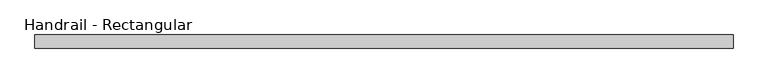
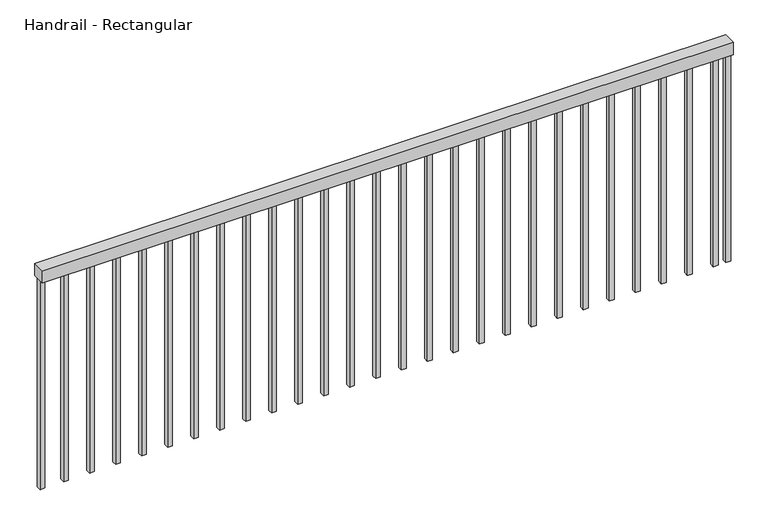
"""IFC4 building model written with IfcOpenShell, lengths in millimetres: railing geometry, Handrail - Rectangular."""

from ifc_helpers import new_model, si_unit, frame, origin, place, context, project, spatial, polyline, outline, extrude, source, transform, mapped, element, save


def handrail_rectangular_428e308a(model_context):
    return source(origin(), model_context, "Body", "SweptSolid", [
        extrude(outline(polyline([(-3385.2211091, 9945.0507146), (-3385.2211091, 9995.8507146), (-685.2211091, 9995.8507146), (-685.2211091, 9945.0507146), (-3385.2211091, 9945.0507146)])), frame((0.0, 0.0, 6654.4), z_axis=(0.0, 0.0, 1.0), x_axis=(1.0, 0.0, 0.0)), (0.0, 0.0, 1.0), 50.8),
        extrude(outline(polyline([(-753.1461091, 9960.9257146), (-753.1461091, 9979.9757146), (-734.0961091, 9979.9757146), (-734.0961091, 9960.9257146), (-753.1461091, 9960.9257146)])), frame((0.0, 0.0, 5790.8), z_axis=(0.0, 0.0, 1.0), x_axis=(1.0, 0.0, 0.0)), (0.0, 0.0, 1.0), 863.6),
        extrude(outline(polyline([(-854.7461091, 9960.9257146), (-854.7461091, 9979.9757146), (-835.6961091, 9979.9757146), (-835.6961091, 9960.9257146), (-854.7461091, 9960.9257146)])), frame((0.0, 0.0, 5790.8), z_axis=(0.0, 0.0, 1.0), x_axis=(1.0, 0.0, 0.0)), (0.0, 0.0, 1.0), 863.6),
        extrude(outline(polyline([(-956.3461091, 9960.9257146), (-956.3461091, 9979.9757146), (-937.2961091, 9979.9757146), (-937.2961091, 9960.9257146), (-956.3461091, 9960.9257146)])), frame((0.0, 0.0, 5790.8), z_axis=(0.0, 0.0, 1.0), x_axis=(1.0, 0.0, 0.0)), (0.0, 0.0, 1.0), 863.6),
        extrude(outline(polyline([(-1057.9461091, 9960.9257146), (-1057.9461091, 9979.9757146), (-1038.8961091, 9979.9757146), (-1038.8961091, 9960.9257146), (-1057.9461091, 9960.9257146)])), frame((0.0, 0.0, 5790.8), z_axis=(0.0, 0.0, 1.0), x_axis=(1.0, 0.0, 0.0)), (0.0, 0.0, 1.0), 863.6),
        extrude(outline(polyline([(-1159.5461091, 9960.9257146), (-1159.5461091, 9979.9757146), (-1140.4961091, 9979.9757146), (-1140.4961091, 9960.9257146), (-1159.5461091, 9960.9257146)])), frame((0.0, 0.0, 5790.8), z_axis=(0.0, 0.0, 1.0), x_axis=(1.0, 0.0, 0.0)), (0.0, 0.0, 1.0), 863.6),
        extrude(outline(polyline([(-1261.1461091, 9960.9257146), (-1261.1461091, 9979.9757146), (-1242.0961091, 9979.9757146), (-1242.0961091, 9960.9257146), (-1261.1461091, 9960.9257146)])), frame((0.0, 0.0, 5790.8), z_axis=(0.0, 0.0, 1.0), x_axis=(1.0, 0.0, 0.0)), (0.0, 0.0, 1.0), 863.6),
        extrude(outline(polyline([(-1362.7461091, 9960.9257146), (-1362.7461091, 9979.9757146), (-1343.6961091, 9979.9757146), (-1343.6961091, 9960.9257146), (-1362.7461091, 9960.9257146)])), frame((0.0, 0.0, 5790.8), z_axis=(0.0, 0.0, 1.0), x_axis=(1.0, 0.0, 0.0)), (0.0, 0.0, 1.0), 863.6),
        extrude(outline(polyline([(-1464.3461091, 9960.9257146), (-1464.3461091, 9979.9757146), (-1445.2961091, 9979.9757146), (-1445.2961091, 9960.9257146), (-1464.3461091, 9960.9257146)])), frame((0.0, 0.0, 5790.8), z_axis=(0.0, 0.0, 1.0), x_axis=(1.0, 0.0, 0.0)), (0.0, 0.0, 1.0), 863.6),
        extrude(outline(polyline([(-1565.9461091, 9960.9257146), (-1565.9461091, 9979.9757146), (-1546.8961091, 9979.9757146), (-1546.8961091, 9960.9257146), (-1565.9461091, 9960.9257146)])), frame((0.0, 0.0, 5790.8), z_axis=(0.0, 0.0, 1.0), x_axis=(1.0, 0.0, 0.0)), (0.0, 0.0, 1.0), 863.6),
        extrude(outline(polyline([(-1667.5461091, 9960.9257146), (-1667.5461091, 9979.9757146), (-1648.4961091, 9979.9757146), (-1648.4961091, 9960.9257146), (-1667.5461091, 9960.9257146)])), frame((0.0, 0.0, 5790.8), z_axis=(0.0, 0.0, 1.0), x_axis=(1.0, 0.0, 0.0)), (0.0, 0.0, 1.0), 863.6),
        extrude(outline(polyline([(-1769.1461091, 9960.9257146), (-1769.1461091, 9979.9757146), (-1750.0961091, 9979.9757146), (-1750.0961091, 9960.9257146), (-1769.1461091, 9960.9257146)])), frame((0.0, 0.0, 5790.8), z_axis=(0.0, 0.0, 1.0), x_axis=(1.0, 0.0, 0.0)), (0.0, 0.0, 1.0), 863.6),
        extrude(outline(polyline([(-1870.7461091, 9960.9257146), (-1870.7461091, 9979.9757146), (-1851.6961091, 9979.9757146), (-1851.6961091, 9960.9257146), (-1870.7461091, 9960.9257146)])), frame((0.0, 0.0, 5790.8), z_axis=(0.0, 0.0, 1.0), x_axis=(1.0, 0.0, 0.0)), (0.0, 0.0, 1.0), 863.6),
        extrude(outline(polyline([(-1972.3461091, 9960.9257146), (-1972.3461091, 9979.9757146), (-1953.2961091, 9979.9757146), (-1953.2961091, 9960.9257146), (-1972.3461091, 9960.9257146)])), frame((0.0, 0.0, 5790.8), z_axis=(0.0, 0.0, 1.0), x_axis=(1.0, 0.0, 0.0)), (0.0, 0.0, 1.0), 863.6),
        extrude(outline(polyline([(-2073.9461091, 9960.9257146), (-2073.9461091, 9979.9757146), (-2054.8961091, 9979.9757146), (-2054.8961091, 9960.9257146), (-2073.9461091, 9960.9257146)])), frame((0.0, 0.0, 5790.8), z_axis=(0.0, 0.0, 1.0), x_axis=(1.0, 0.0, 0.0)), (0.0, 0.0, 1.0), 863.6),
        extrude(outline(polyline([(-2175.5461091, 9960.9257146), (-2175.5461091, 9979.9757146), (-2156.4961091, 9979.9757146), (-2156.4961091, 9960.9257146), (-2175.5461091, 9960.9257146)])), frame((0.0, 0.0, 5790.8), z_axis=(0.0, 0.0, 1.0), x_axis=(1.0, 0.0, 0.0)), (0.0, 0.0, 1.0), 863.6),
        extrude(outline(polyline([(-2277.1461091, 9960.9257146), (-2277.1461091, 9979.9757146), (-2258.0961091, 9979.9757146), (-2258.0961091, 9960.9257146), (-2277.1461091, 9960.9257146)])), frame((0.0, 0.0, 5790.8), z_axis=(0.0, 0.0, 1.0), x_axis=(1.0, 0.0, 0.0)), (0.0, 0.0, 1.0), 863.6),
        extrude(outline(polyline([(-2378.7461091, 9960.9257146), (-2378.7461091, 9979.9757146), (-2359.6961091, 9979.9757146), (-2359.6961091, 9960.9257146), (-2378.7461091, 9960.9257146)])), frame((0.0, 0.0, 5790.8), z_axis=(0.0, 0.0, 1.0), x_axis=(1.0, 0.0, 0.0)), (0.0, 0.0, 1.0), 863.6),
        extrude(outline(polyline([(-2480.3461091, 9960.9257146), (-2480.3461091, 9979.9757146), (-2461.2961091, 9979.9757146), (-2461.2961091, 9960.9257146), (-2480.3461091, 9960.9257146)])), frame((0.0, 0.0, 5790.8), z_axis=(0.0, 0.0, 1.0), x_axis=(1.0, 0.0, 0.0)), (0.0, 0.0, 1.0), 863.6),
        extrude(outline(polyline([(-2581.9461091, 9960.9257146), (-2581.9461091, 9979.9757146), (-2562.8961091, 9979.9757146), (-2562.8961091, 9960.9257146), (-2581.9461091, 9960.9257146)])), frame((0.0, 0.0, 5790.8), z_axis=(0.0, 0.0, 1.0), x_axis=(1.0, 0.0, 0.0)), (0.0, 0.0, 1.0), 863.6),
        extrude(outline(polyline([(-2683.5461091, 9960.9257146), (-2683.5461091, 9979.9757146), (-2664.4961091, 9979.9757146), (-2664.4961091, 9960.9257146), (-2683.5461091, 9960.9257146)])), frame((0.0, 0.0, 5790.8), z_axis=(0.0, 0.0, 1.0), x_axis=(1.0, 0.0, 0.0)), (0.0, 0.0, 1.0), 863.6),
        extrude(outline(polyline([(-2785.1461091, 9960.9257146), (-2785.1461091, 9979.9757146), (-2766.0961091, 9979.9757146), (-2766.0961091, 9960.9257146), (-2785.1461091, 9960.9257146)])), frame((0.0, 0.0, 5790.8), z_axis=(0.0, 0.0, 1.0), x_axis=(1.0, 0.0, 0.0)), (0.0, 0.0, 1.0), 863.6),
        extrude(outline(polyline([(-2886.7461091, 9960.9257146), (-2886.7461091, 9979.9757146), (-2867.6961091, 9979.9757146), (-2867.6961091, 9960.9257146), (-2886.7461091, 9960.9257146)])), frame((0.0, 0.0, 5790.8), z_axis=(0.0, 0.0, 1.0), x_axis=(1.0, 0.0, 0.0)), (0.0, 0.0, 1.0), 863.6),
        extrude(outline(polyline([(-2988.3461091, 9960.9257146), (-2988.3461091, 9979.9757146), (-2969.2961091, 9979.9757146), (-2969.2961091, 9960.9257146), (-2988.3461091, 9960.9257146)])), frame((0.0, 0.0, 5790.8), z_axis=(0.0, 0.0, 1.0), x_axis=(1.0, 0.0, 0.0)), (0.0, 0.0, 1.0), 863.6),
        extrude(outline(polyline([(-3089.9461091, 9960.9257146), (-3089.9461091, 9979.9757146), (-3070.8961091, 9979.9757146), (-3070.8961091, 9960.9257146), (-3089.9461091, 9960.9257146)])), frame((0.0, 0.0, 5790.8), z_axis=(0.0, 0.0, 1.0), x_axis=(1.0, 0.0, 0.0)), (0.0, 0.0, 1.0), 863.6),
        extrude(outline(polyline([(-3191.5461091, 9960.9257146), (-3191.5461091, 9979.9757146), (-3172.4961091, 9979.9757146), (-3172.4961091, 9960.9257146), (-3191.5461091, 9960.9257146)])), frame((0.0, 0.0, 5790.8), z_axis=(0.0, 0.0, 1.0), x_axis=(1.0, 0.0, 0.0)), (0.0, 0.0, 1.0), 863.6),
        extrude(outline(polyline([(-3293.1461091, 9960.9257146), (-3293.1461091, 9979.9757146), (-3274.0961091, 9979.9757146), (-3274.0961091, 9960.9257146), (-3293.1461091, 9960.9257146)])), frame((0.0, 0.0, 5790.8), z_axis=(0.0, 0.0, 1.0), x_axis=(1.0, 0.0, 0.0)), (0.0, 0.0, 1.0), 863.6),
        extrude(outline(polyline([(-704.2711091, 9960.9257146), (-704.2711091, 9979.9757146), (-685.2211091, 9979.9757146), (-685.2211091, 9960.9257146), (-704.2711091, 9960.9257146)])), frame((0.0, 0.0, 5790.8), z_axis=(0.0, 0.0, 1.0), x_axis=(1.0, 0.0, 0.0)), (0.0, 0.0, 1.0), 863.6),
        extrude(outline(polyline([(-3385.2211091, 9960.9257146), (-3385.2211091, 9979.9757146), (-3366.1711091, 9979.9757146), (-3366.1711091, 9960.9257146), (-3385.2211091, 9960.9257146)])), frame((0.0, 0.0, 5790.8), z_axis=(0.0, 0.0, 1.0), x_axis=(1.0, 0.0, 0.0)), (0.0, 0.0, 1.0), 863.6),
    ])


if __name__ == "__main__":
    model = new_model("IFC4")
    model_context = context("Model", 3, world=origin())
    ifc_project = project(units=[si_unit("LENGTHUNIT", "METRE", prefix="MILLI")], contexts=[model_context])
    site = spatial("IfcSite", under=ifc_project)
    building = spatial("IfcBuilding", under=site)
    placement = place(None, origin())
    handrail_rectangular_shape = handrail_rectangular_428e308a(model_context)
    element("IfcRailing", 1, ObjectType="Handrail - Rectangular", at=placement, inside=building, context=model_context, shape_type="MappedRepresentation", body=[
        mapped(handrail_rectangular_shape, transform((0.0, 0.0, 0.0), x_axis=(1.0, 0.0, 0.0), y_axis=(0.0, 1.0, 0.0), z_axis=(0.0, 0.0, 1.0))),
    ])
    save(model, "model.ifc")
